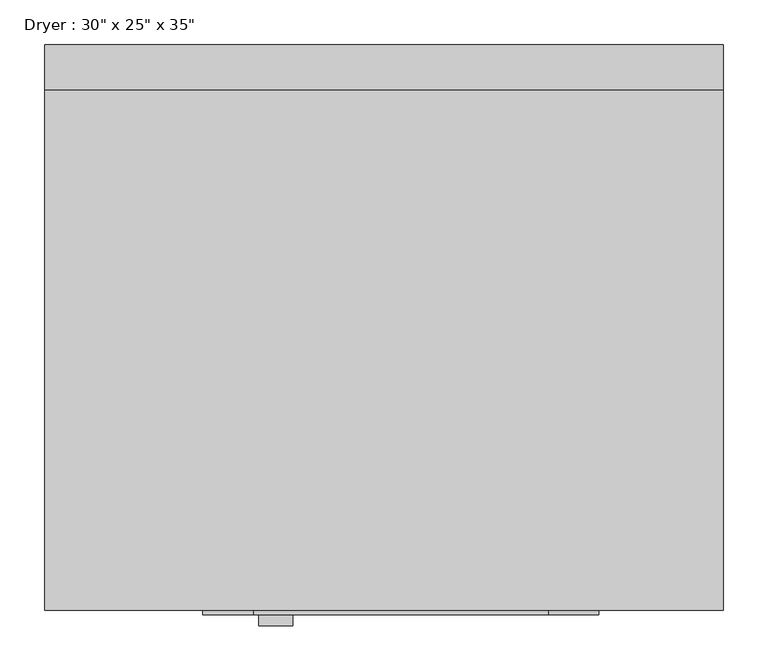
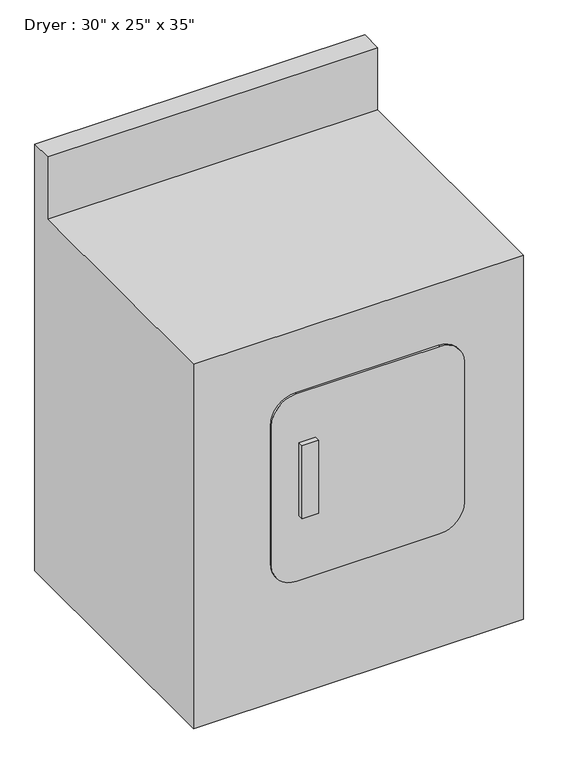
"""IFC4 building model written with IfcOpenShell, lengths in millimetres: proxy geometry."""

from ifc_helpers import new_model, si_unit, point, frame, frame_2d, origin, place, context, project, spatial, polyline, circle_curve, trimmed, segment, composite_curve, outline, extrude, source, transform, mapped, element, save


def proxy_6b4a07a9(model_context):
    return source(origin(), model_context, "Body", "SweptSolid", [
        extrude(outline(polyline([(314.8635206, -20.3014962), (276.7635206, -20.3014962), (276.7635206, -7.6014962), (314.8635206, -7.6014962), (314.8635206, -20.3014962)])), frame((0.0, 0.0, 438.7649313), z_axis=(0.0, 0.0, 1.0), x_axis=(1.0, 0.0, 0.0)), (0.0, 0.0, 1.0), 177.8),
        extrude(outline(composite_curve([segment(polyline([(737.623844, 601.2374563), (737.623844, 271.0374563)]), True, "CONTINUOUS"), segment(trimmed(circle_curve(frame_2d((680.473844, 271.0374563)), 57.15), [point((737.623844, 271.0374563))], [point((680.473844, 213.8874563))], False, "CARTESIAN"), True, "CONTINUOUS"), segment(polyline([(680.473844, 213.8874563), (337.573844, 213.8874563)]), True, "CONTINUOUS"), segment(trimmed(circle_curve(frame_2d((337.573844, 271.0374563)), 57.15), [point((337.573844, 213.8874563))], [point((280.423844, 271.0374563))], False, "CARTESIAN"), True, "CONTINUOUS"), segment(polyline([(280.423844, 271.0374563), (280.423844, 601.2374563)]), True, "CONTINUOUS"), segment(trimmed(circle_curve(frame_2d((337.573844, 601.2374563)), 57.15), [point((280.423844, 601.2374563))], [point((337.573844, 658.3874563))], False, "CARTESIAN"), True, "CONTINUOUS"), segment(polyline([(337.573844, 658.3874563), (680.473844, 658.3874563)]), True, "CONTINUOUS"), segment(trimmed(circle_curve(frame_2d((680.473844, 601.2374563)), 57.15), [point((680.473844, 658.3874563))], [point((737.623844, 601.2374563))], False, "CARTESIAN"), True, "CONTINUOUS")], self_intersect=False)), frame((0.0, -7.6014962, 0.0), z_axis=(0.0, 1.0, 0.0), x_axis=(0.0, 0.0, 1.0)), (0.0, 0.0, 1.0), 4.7625),
        extrude(outline(polyline([(632.1610038, 0.0), (-2.8389962, 0.0), (-2.8389962, 889.0), (581.3610038, 889.0), (581.3610038, 1041.4), (632.1610038, 1041.4), (632.1610038, 0.0)])), frame((36.0874563, 0.0, 0.0), z_axis=(1.0, 0.0, 0.0), x_axis=(0.0, 1.0, 0.0)), (0.0, 0.0, 1.0), 762.0),
    ])


if __name__ == "__main__":
    model = new_model("IFC4")
    model_context = context("Model", 3, world=origin())
    ifc_project = project(units=[si_unit("LENGTHUNIT", "METRE", prefix="MILLI")], contexts=[model_context])
    site = spatial("IfcSite", under=ifc_project)
    building = spatial("IfcBuilding", under=site)
    placement = place(None, origin())
    proxy_shape = proxy_6b4a07a9(model_context)
    element("IfcBuildingElementProxy", 1, Name="Dryer : 30\" x 25\" x 35\"", ObjectType="Dryer : 30\" x 25\" x 35\"", at=placement, inside=building, context=model_context, shape_type="MappedRepresentation", body=[
        mapped(proxy_shape, transform((0.0, 0.0, 0.0), x_axis=(1.0, 0.0, 0.0), y_axis=(0.0, 1.0, 0.0), z_axis=(0.0, 0.0, 1.0))),
    ])
    save(model, "model.ifc")

# Revit data of these elements
# Type "Dryer : 30\" x 25\" x 35\""
#   Label = "D"
#   Assembly Code = "E1090400"
#   Depth = 2' - 1"
#   Height = 2' - 11"
#   Width = 2' - 6"
#   Dryer Material = Steel, Paint Finish, Ivory, Glossy
#   Default Elevation = 0
# Element 1 (IfcBuildingElementProxy, "Dryer : 30\" x 25\" x 35\"")
#   Materials on its faces: "Steel, Paint Finish, Ivory, Glossy"
# Materials
#   "Steel, Paint Finish, Ivory, Glossy": class "Metal", colour RGB 242 242 229, transparency 0, Description = "Steel, paint finish, ivory, glossy", Cost = 0
